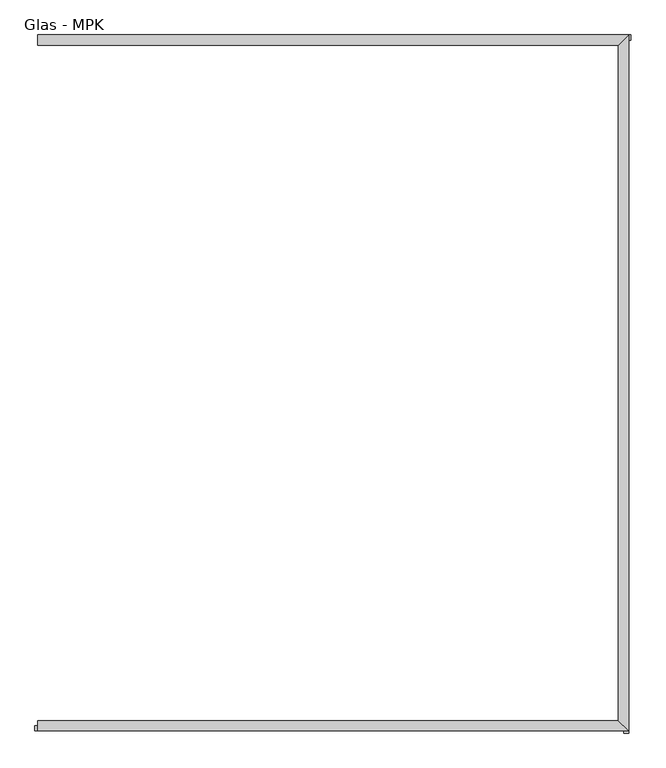
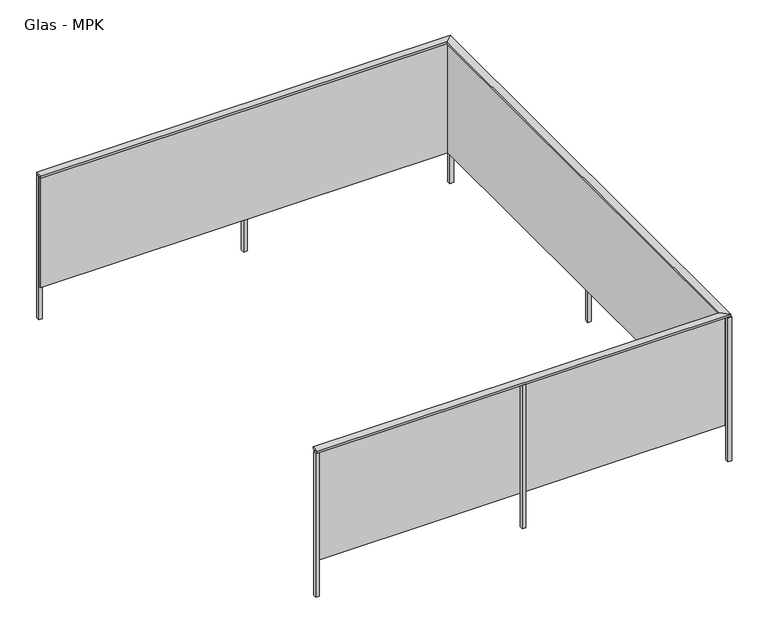
"""IFC4 building model written with IfcOpenShell, lengths in millimetres: railing geometry, Glas - MPK."""

from ifc_helpers import new_model, si_unit, frame, origin, place, context, project, spatial, polyline, outline, extrude, faceted_brep, source, transform, mapped, element, save


def glas_mpk_389492d2(model_context):
    return source(origin(), model_context, "Body", "SolidModel", [
        faceted_brep([(28820.4268037, 1294.9571597, 12843.2628643), (28820.4268037, 1244.9571597, 12843.2628643), (28820.4268037, 1244.9571597, 12856.7371357), (28820.4268037, 1294.9571597, 12856.7371357), (31660.4268037, 1294.9571597, 12843.2628643), (31610.4268037, 1244.9571597, 12843.2628643), (31610.4268037, 1244.9571597, 12856.7371357), (31660.4268037, 1294.9571597, 12856.7371357), (31660.4268037, -2045.7721864, 12843.2628643), (31610.4268037, -1995.7721864, 12843.2628643), (31610.4268037, -1995.7721864, 12856.7371357), (31660.4268037, -2045.7721864, 12856.7371357), (28820.4268037, -2045.7721864, 12843.2628643), (28820.4268037, -2045.7721864, 12856.7371357), (28820.4268037, -1995.7721864, 12856.7371357), (28820.4268037, -1995.7721864, 12843.2628643)], [[[0, 1, 2, 3]], [[1, 0, 4, 5]], [[2, 1, 5, 6]], [[3, 2, 6, 7]], [[0, 3, 7, 4]], [[5, 4, 8, 9]], [[6, 5, 9, 10]], [[7, 6, 10, 11]], [[4, 7, 11, 8]], [[12, 13, 14, 15]], [[9, 8, 12, 15]], [[10, 9, 15, 14]], [[11, 10, 14, 13]], [[8, 11, 13, 12]]]),
        faceted_brep([(28820.4268037, 1254.9571597, 12842.8769824), (28820.4268037, 1269.1492837, 12842.8769824), (28820.4268037, 1269.1492837, 12042.8769824), (28820.4268037, 1254.9571597, 12042.8769824), (31620.4268037, 1254.9571597, 12842.8769824), (31634.6189277, 1269.1492837, 12842.8769824), (31634.6189277, 1269.1492837, 12042.8769824), (31620.4268037, 1254.9571597, 12042.8769824), (31620.4268037, -2005.7721864, 12842.8769824), (31634.6189277, -2019.9643104, 12842.8769824), (31634.6189277, -2019.9643104, 12042.8769824), (31620.4268037, -2005.7721864, 12042.8769824), (28820.4268037, -2005.7721864, 12842.8769824), (28820.4268037, -2005.7721864, 12042.8769824), (28820.4268037, -2019.9643104, 12042.8769824), (28820.4268037, -2019.9643104, 12842.8769824)], [[[0, 1, 2, 3]], [[1, 0, 4, 5]], [[2, 1, 5, 6]], [[3, 2, 6, 7]], [[0, 3, 7, 4]], [[5, 4, 8, 9]], [[6, 5, 9, 10]], [[7, 6, 10, 11]], [[4, 7, 11, 8]], [[12, 13, 14, 15]], [[9, 8, 12, 15]], [[10, 9, 15, 14]], [[11, 10, 14, 13]], [[8, 11, 13, 12]]]),
        extrude(outline(polyline([(30251.6768037, -2020.7721864), (30251.6768037, -2045.7721864), (30226.6768037, -2045.7721864), (30226.6768037, -2020.7721864), (30251.6768037, -2020.7721864)])), frame((0.0, 0.0, 11800.0), z_axis=(0.0, 0.0, 1.0), x_axis=(1.0, 0.0, 0.0)), (0.0, 0.0, 1.0), 1043.2628643),
        extrude(outline(polyline([(31635.4268037, -362.9075133), (31660.4268037, -362.9075133), (31660.4268037, -387.9075133), (31635.4268037, -387.9075133), (31635.4268037, -362.9075133)])), frame((0.0, 0.0, 11800.0), z_axis=(0.0, 0.0, 1.0), x_axis=(1.0, 0.0, 0.0)), (0.0, 0.0, 1.0), 1043.2628643),
        extrude(outline(polyline([(30226.6768037, 1269.9571597), (30226.6768037, 1294.9571597), (30251.6768037, 1294.9571597), (30251.6768037, 1269.9571597), (30226.6768037, 1269.9571597)])), frame((0.0, 0.0, 11800.0), z_axis=(0.0, 0.0, 1.0), x_axis=(1.0, 0.0, 0.0)), (0.0, 0.0, 1.0), 1043.2628643),
        extrude(outline(polyline([(31635.4268037, -2030.7721864), (31660.4268037, -2030.7721864), (31660.4268037, -2055.7721864), (31635.4268037, -2055.7721864), (31635.4268037, -2030.7721864)])), frame((0.0, 0.0, 11800.0), z_axis=(0.0, 0.0, 1.0), x_axis=(1.0, 0.0, 0.0)), (0.0, 0.0, 1.0), 1043.2628643),
        extrude(outline(polyline([(31645.4268037, 1269.9571597), (31645.4268037, 1294.9571597), (31670.4268037, 1294.9571597), (31670.4268037, 1269.9571597), (31645.4268037, 1269.9571597)])), frame((0.0, 0.0, 11800.0), z_axis=(0.0, 0.0, 1.0), x_axis=(1.0, 0.0, 0.0)), (0.0, 0.0, 1.0), 1043.2628643),
        extrude(outline(polyline([(28832.9268037, -2020.7721864), (28832.9268037, -2045.7721864), (28807.9268037, -2045.7721864), (28807.9268037, -2020.7721864), (28832.9268037, -2020.7721864)])), frame((0.0, 0.0, 11800.0), z_axis=(0.0, 0.0, 1.0), x_axis=(1.0, 0.0, 0.0)), (0.0, 0.0, 1.0), 1043.2628643),
        extrude(outline(polyline([(28820.4268037, 1269.9571597), (28820.4268037, 1294.9571597), (28845.4268037, 1294.9571597), (28845.4268037, 1269.9571597), (28820.4268037, 1269.9571597)])), frame((0.0, 0.0, 11800.0), z_axis=(0.0, 0.0, 1.0), x_axis=(1.0, 0.0, 0.0)), (0.0, 0.0, 1.0), 1043.2628643),
    ])


if __name__ == "__main__":
    model = new_model("IFC4")
    model_context = context("Model", 3, world=origin())
    ifc_project = project(units=[si_unit("LENGTHUNIT", "METRE", prefix="MILLI")], contexts=[model_context])
    site = spatial("IfcSite", under=ifc_project)
    building = spatial("IfcBuilding", under=site)
    placement = place(None, origin())
    glas_mpk_shape = glas_mpk_389492d2(model_context)
    element("IfcRailing", 1, ObjectType="Glas - MPK", at=placement, inside=building, context=model_context, shape_type="MappedRepresentation", body=[
        mapped(glas_mpk_shape, transform((0.0, 0.0, 0.0), x_axis=(1.0, 0.0, 0.0), y_axis=(0.0, 1.0, 0.0), z_axis=(0.0, 0.0, 1.0))),
    ])
    save(model, "model.ifc")

# Revit data of these elements
# Element 1 (IfcRailing, "Glas - MPK")
#   Materials on its faces: "Metal - Aluminum", "Window - Glass"
# Materials
#   "Metal - Aluminum": class "Unassigned", colour RGB 247 247 247, transparency 0, Comments = "Rendering appearance not upgraded "
#   "Window - Glass": class "Glas", colour RGB 128 128 255, transparency 0.75
